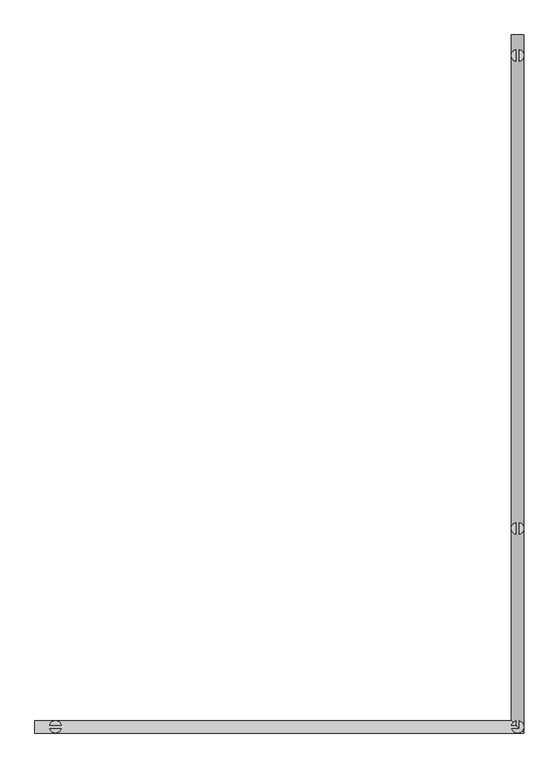
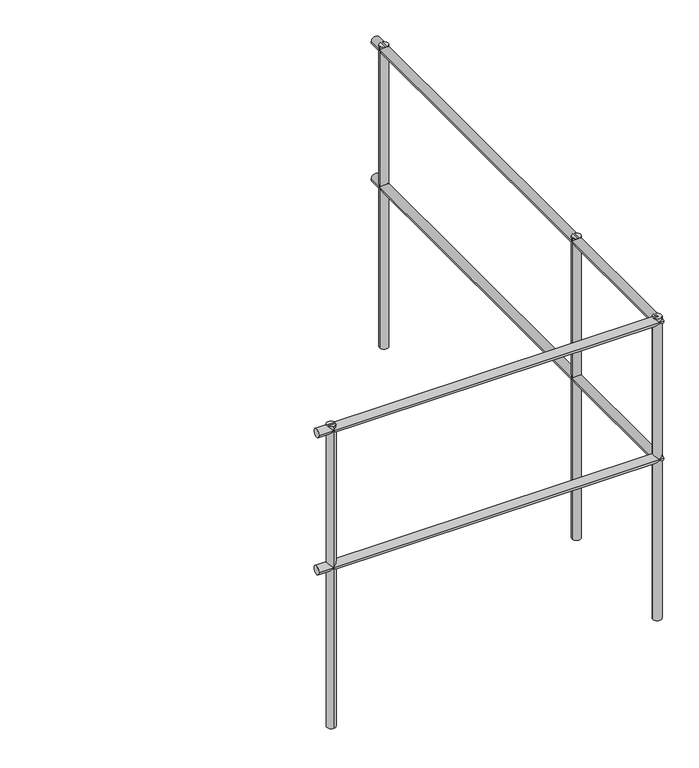
"""IFC4 building model written with IfcOpenShell, lengths in millimetres: railing geometry."""

from ifc_helpers import new_model, si_unit, point, frame, frame_2d, origin, place, context, project, spatial, circle_curve, ellipse_curve, trimmed, segment, composite_curve, outline, extrude, source, transform, mapped, element, save
from ifc_brep_helpers import plane_surface, cylinder_surface, advanced_brep


def railing_1ae78489(model_context):
    return source(origin(), model_context, "Body", "SolidModel", [
        advanced_brep(
        [(11414.7052251, 14979.5208589, 5045.0), (11384.7052251, 14979.5208589, 5045.0), (10225.0, 13282.0208589, 5045.0), (10225.0, 13312.0208589, 5045.0), (11414.7052251, 13282.0208589, 5045.0), (11384.7052251, 13312.0208589, 5045.0)],
        [
            (0, 1, circle_curve(frame((11399.7052251, 14979.5208589, 5045.0), z_axis=(0.0, 1.0, 0.0), x_axis=(-1.0, 0.0, 0.0)), 15.0)),
            (1, 0, circle_curve(frame((11399.7052251, 14979.5208589, 5045.0), z_axis=(0.0, 1.0, 0.0), x_axis=(-1.0, 0.0, 0.0)), 15.0)),
            (2, 3, circle_curve(frame((10225.0, 13297.0208589, 5045.0), z_axis=(-1.0, 0.0, 0.0), x_axis=(0.0, 1.0, 0.0)), 15.0)),
            (3, 2, circle_curve(frame((10225.0, 13297.0208589, 5045.0), z_axis=(-1.0, 0.0, 0.0), x_axis=(0.0, 1.0, 0.0)), 15.0)),
            (0, 4),
            (4, 5, ellipse_curve(frame((11399.7052251, 13297.0208589, 5045.0), z_axis=(0.7071067811865475, 0.7071067811865475, 0.0), x_axis=(-0.7071067811865474, 0.7071067811865476, 0.0)), 21.2132034, 15.0)),
            (5, 1),
            (5, 4, ellipse_curve(frame((11399.7052251, 13297.0208589, 5045.0), z_axis=(0.7071067811865475, 0.7071067811865475, 0.0), x_axis=(-0.7071067811865474, 0.7071067811865476, 0.0)), 21.2132034, 15.0)),
            (4, 2),
            (3, 5),
        ],
        [
            plane_surface(frame((11399.7052251, 14979.5208589, 5060.0), z_axis=(0.0, 1.0, 0.0), x_axis=(0.0, 0.0, -1.0))),
            plane_surface(frame((10225.0, 13297.0208589, 5060.0), z_axis=(-1.0, 0.0, 0.0), x_axis=(0.0, -1.0, 0.0))),
            cylinder_surface(frame((11399.7052251, 14979.5208589, 5045.0), z_axis=(0.0, 1.0, 0.0), x_axis=(-1.0, 0.0, 0.0)), 15.0),
            cylinder_surface(frame((11399.7052251, 13297.0208589, 5045.0), z_axis=(1.0, 0.0, 0.0), x_axis=(0.0, 1.0, 0.0)), 15.0),
        ],
        [
            (0, [[1, 2]]),
            (1, [[3, 4]]),
            (2, [[-1, 5, 6, 7]]),
            (2, [[-2, -7, 8, -5]]),
            (3, [[-6, 9, -4, 10]]),
            (3, [[-8, -10, -3, -9]]),
        ],
    ),
        advanced_brep(
        [(11414.7052251, 14979.5208589, 5545.0), (11384.7052251, 14979.5208589, 5545.0), (11414.7052251, 13282.0208589, 5545.0), (11384.7052251, 13312.0208589, 5545.0), (10225.0, 13282.0208589, 5545.0), (10225.0, 13312.0208589, 5545.0)],
        [
            (0, 1, circle_curve(frame((11399.7052251, 14979.5208589, 5545.0), z_axis=(0.0, 1.0, 0.0), x_axis=(-1.0, 0.0, 0.0)), 15.0)),
            (1, 0, circle_curve(frame((11399.7052251, 14979.5208589, 5545.0), z_axis=(0.0, 1.0, 0.0), x_axis=(-1.0, 0.0, 0.0)), 15.0)),
            (0, 2),
            (2, 3, ellipse_curve(frame((11399.7052251, 13297.0208589, 5545.0), z_axis=(0.7071067811865475, 0.7071067811865475, 0.0), x_axis=(-0.7071067811865474, 0.7071067811865476, 0.0)), 21.2132034, 15.0)),
            (3, 1),
            (3, 2, ellipse_curve(frame((11399.7052251, 13297.0208589, 5545.0), z_axis=(0.7071067811865475, 0.7071067811865475, 0.0), x_axis=(-0.7071067811865474, 0.7071067811865476, 0.0)), 21.2132034, 15.0)),
            (4, 5, circle_curve(frame((10225.0, 13297.0208589, 5545.0), z_axis=(-1.0, 0.0, 0.0), x_axis=(0.0, 1.0, 0.0)), 15.0)),
            (5, 4, circle_curve(frame((10225.0, 13297.0208589, 5545.0), z_axis=(-1.0, 0.0, 0.0), x_axis=(0.0, 1.0, 0.0)), 15.0)),
            (2, 4),
            (5, 3),
        ],
        [
            plane_surface(frame((11399.7052251, 14979.5208589, 5560.0), z_axis=(0.0, 1.0, 0.0), x_axis=(0.0, 0.0, -1.0))),
            cylinder_surface(frame((11399.7052251, 14979.5208589, 5545.0), z_axis=(0.0, 1.0, 0.0), x_axis=(-1.0, 0.0, 0.0)), 15.0),
            plane_surface(frame((10225.0, 13297.0208589, 5560.0), z_axis=(-1.0, 0.0, 0.0), x_axis=(0.0, -1.0, 0.0))),
            cylinder_surface(frame((11399.7052251, 13297.0208589, 5545.0), z_axis=(1.0, 0.0, 0.0), x_axis=(0.0, 1.0, 0.0)), 15.0),
        ],
        [
            (0, [[1, 2]]),
            (1, [[-1, 3, 4, 5]]),
            (1, [[-2, -5, 6, -3]]),
            (2, [[7, 8]]),
            (3, [[-4, 9, -8, 10]]),
            (3, [[-6, -10, -7, -9]]),
        ],
    ),
        extrude(outline(composite_curve([segment(trimmed(circle_curve(frame_2d((11399.7052251, 13779.5208589)), 15.0), [point((11384.7052251, 13779.5208589))], [point((11414.7052251, 13779.5208589))], False, "CARTESIAN"), True, "CONTINUOUS"), segment(trimmed(circle_curve(frame_2d((11399.7052251, 13779.5208589)), 15.0), [point((11414.7052251, 13779.5208589))], [point((11384.7052251, 13779.5208589))], False, "CARTESIAN"), True, "CONTINUOUS")], self_intersect=False)), frame((0.0, 0.0, 4460.0), z_axis=(0.0, 0.0, 1.0), x_axis=(1.0, 0.0, 0.0)), (0.0, 0.0, 1.0), 1100.0),
        extrude(outline(composite_curve([segment(trimmed(circle_curve(frame_2d((11399.7052251, 13297.0208589)), 15.0), [point((11384.7052251, 13297.0208589))], [point((11414.7052251, 13297.0208589))], False, "CARTESIAN"), True, "CONTINUOUS"), segment(trimmed(circle_curve(frame_2d((11399.7052251, 13297.0208589)), 15.0), [point((11414.7052251, 13297.0208589))], [point((11384.7052251, 13297.0208589))], False, "CARTESIAN"), True, "CONTINUOUS")], self_intersect=False)), frame((0.0, 0.0, 4460.0), z_axis=(0.0, 0.0, 1.0), x_axis=(1.0, 0.0, 0.0)), (0.0, 0.0, 1.0), 1100.0),
        extrude(outline(composite_curve([segment(trimmed(circle_curve(frame_2d((10275.0, 13297.0208589)), 15.0), [point((10275.0, 13312.0208589))], [point((10275.0, 13282.0208589))], False, "CARTESIAN"), True, "CONTINUOUS"), segment(trimmed(circle_curve(frame_2d((10275.0, 13297.0208589)), 15.0), [point((10275.0, 13282.0208589))], [point((10275.0, 13312.0208589))], False, "CARTESIAN"), True, "CONTINUOUS")], self_intersect=False)), frame((0.0, 0.0, 4460.0), z_axis=(0.0, 0.0, 1.0), x_axis=(1.0, 0.0, 0.0)), (0.0, 0.0, 1.0), 1100.0),
        extrude(outline(composite_curve([segment(trimmed(circle_curve(frame_2d((11399.7052251, 14929.5208589)), 15.0), [point((11384.7052251, 14929.5208589))], [point((11414.7052251, 14929.5208589))], False, "CARTESIAN"), True, "CONTINUOUS"), segment(trimmed(circle_curve(frame_2d((11399.7052251, 14929.5208589)), 15.0), [point((11414.7052251, 14929.5208589))], [point((11384.7052251, 14929.5208589))], False, "CARTESIAN"), True, "CONTINUOUS")], self_intersect=False)), frame((0.0, 0.0, 4460.0), z_axis=(0.0, 0.0, 1.0), x_axis=(1.0, 0.0, 0.0)), (0.0, 0.0, 1.0), 1100.0),
    ])


if __name__ == "__main__":
    model = new_model("IFC4")
    model_context = context("Model", 3, world=origin())
    ifc_project = project(units=[si_unit("LENGTHUNIT", "METRE", prefix="MILLI")], contexts=[model_context])
    site = spatial("IfcSite", under=ifc_project)
    building = spatial("IfcBuilding", under=site)
    placement = place(None, origin())
    railing_shape = railing_1ae78489(model_context)
    element("IfcRailing", 1, at=placement, inside=building, context=model_context, shape_type="MappedRepresentation", body=[
        mapped(railing_shape, transform((0.0, 0.0, 0.0), x_axis=(1.0, 0.0, 0.0), y_axis=(0.0, 1.0, 0.0), z_axis=(0.0, 0.0, 1.0))),
    ])
    save(model, "model.ifc")
